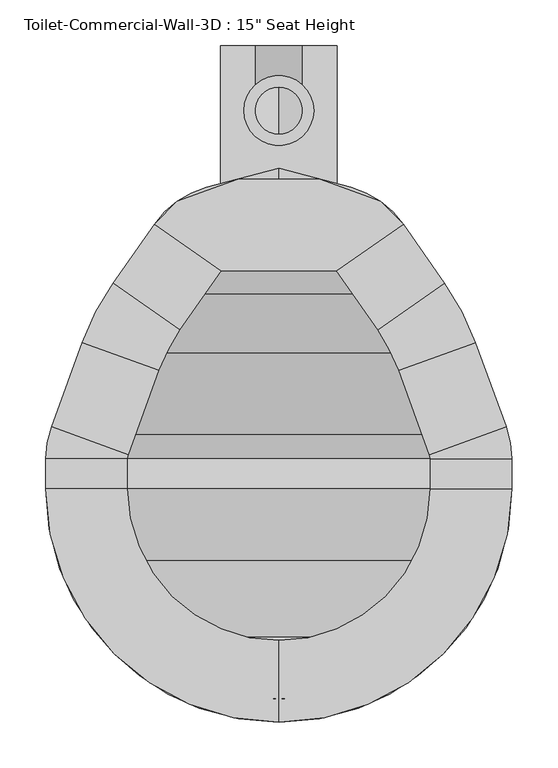
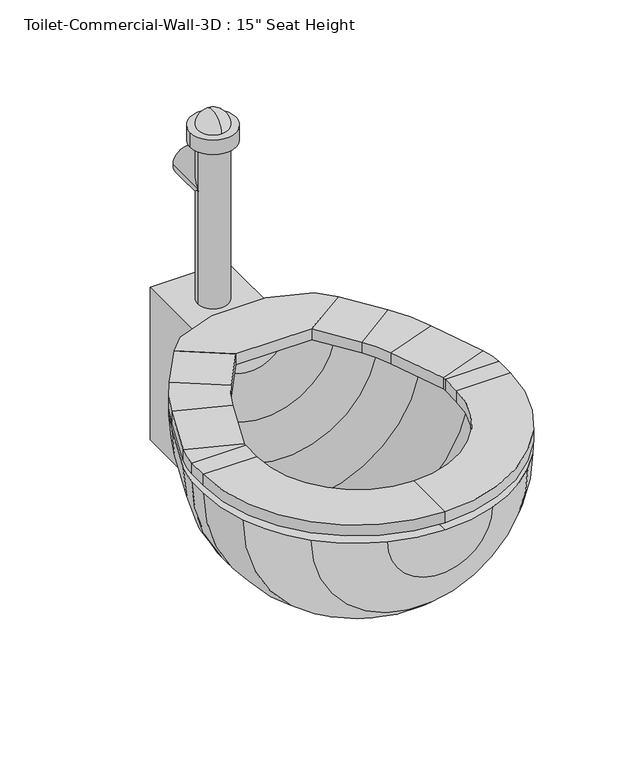
"""IFC4 building model written with IfcOpenShell, lengths in millimetres: flow terminal geometry."""

import ifcopenshell
import ifcopenshell.guid

model = None  # the IFC model being written
_history = None  # IfcOwnerHistory: only IFC2X3 demands one
_inside = {}  # id of a spatial element -> (the spatial element, [elements in it])
_under = {}  # id of a project, library or spatial element -> (it, [spatial elements below it])
_declared = {}  # id of a project -> (the project, [libraries it declares])
_typed = {}  # id of a type object -> (the type object, [elements of that type])
_made_of = {}  # id of a material, layer set ... -> (it, [elements and type objects made of it])


def new_model(schema):
    """Start an empty IFC model of exactly this schema.

    Asked for "IFC4X3", IfcOpenShell would pick the latest addendum, in which some entities
    have other attributes; the version numbers below select the first issue.
    IFC2X3 requires an IfcOwnerHistory on every rooted entity: one is made here for all.
    """
    global model, _history
    if schema == "IFC4X3":
        model = ifcopenshell.file(schema_version=(4, 3, 0, 0))
    else:
        model = ifcopenshell.file(schema=schema)
    _inside.clear()
    _under.clear()
    _declared.clear()
    _typed.clear()
    _made_of.clear()
    _history = None
    if model.schema == "IFC2X3":
        org = make("IfcOrganization", Name="unknown")
        user = make(
            "IfcPersonAndOrganization",
            ThePerson=make("IfcPerson", FamilyName="unknown"),
            TheOrganization=org,
        )
        app = make(
            "IfcApplication",
            ApplicationDeveloper=org,
            Version="unknown",
            ApplicationFullName="unknown",
            ApplicationIdentifier="unknown",
        )
        _history = make(
            "IfcOwnerHistory",
            OwningUser=user,
            OwningApplication=app,
            ChangeAction="ADDED",
            CreationDate=0,
        )
    return model


def make(cls, **values):
    """One entity of the class cls with the attributes given. An attribute that is None is left unset."""
    return model.create_entity(
        cls, **{name: value for name, value in values.items() if value is not None}
    )


def rooted(cls, **values):
    """An entity with a GlobalId (a new one), such as an element, a storey or a relation."""
    return make(cls, GlobalId=ifcopenshell.guid.new(), OwnerHistory=_history, **values)


def si_unit(unit_type, name, prefix=None):
    """IfcSIUnit, for example si_unit("LENGTHUNIT", "METRE", prefix="MILLI")."""
    return make("IfcSIUnit", UnitType=unit_type, Prefix=prefix, Name=name)


def assignment(units):
    """IfcUnitAssignment: the units of a project."""
    return None if units is None else make("IfcUnitAssignment", Units=units)


def point(xyz):
    """IfcCartesianPoint."""
    return None if xyz is None else make("IfcCartesianPoint", Coordinates=xyz)


def direction(xyz):
    """IfcDirection."""
    return None if xyz is None else make("IfcDirection", DirectionRatios=xyz)


def frame(location, z_axis=None, x_axis=None):
    """IfcAxis2Placement3D, a coordinate frame: its origin and axes. An axis left out is left unset."""
    return make(
        "IfcAxis2Placement3D",
        Location=point(location),
        Axis=direction(z_axis),
        RefDirection=direction(x_axis),
    )


def frame_2d(location, x_axis=None):
    """IfcAxis2Placement2D, a coordinate frame in the plane: its origin and x axis."""
    return make(
        "IfcAxis2Placement2D", Location=point(location), RefDirection=direction(x_axis)
    )


def origin():
    """The frame at (0, 0, 0) with its axes left unset."""
    return frame((0.0, 0.0, 0.0))


def place(relative_to, where):
    """IfcLocalPlacement: puts the frame where relative to a parent placement (None: the world)."""
    return make(
        "IfcLocalPlacement", PlacementRelTo=relative_to, RelativePlacement=where
    )


def context(
    kind, dimensions, precision=None, world=None, true_north=None, identifier=None
):
    """IfcGeometricRepresentationContext, for example the 3D "Model" context."""
    return make(
        "IfcGeometricRepresentationContext",
        ContextIdentifier=identifier,
        ContextType=kind,
        CoordinateSpaceDimension=dimensions,
        Precision=precision,
        WorldCoordinateSystem=world,
        TrueNorth=true_north,
    )


def project(units=None, contexts=None):
    """IfcProject with its units and contexts."""
    return rooted(
        "IfcProject",
        Name="project",
        RepresentationContexts=contexts,
        UnitsInContext=assignment(units),
    )


def spatial(cls, under=None, at=None, **own):
    """A site, building, storey or space (cls), placed at a placement, below another one or the project."""
    s = rooted(cls, ObjectPlacement=at, **own)
    if under is not None:
        _under.setdefault(under.id(), (under, []))[1].append(s)
    return s


def polyline(points):
    """IfcPolyline through the points."""
    return make("IfcPolyline", Points=[point(p) for p in points])


def circle_curve(where, radius):
    """IfcCircle in the frame where."""
    return make("IfcCircle", Position=where, Radius=radius)


def ellipse_curve(where, semi_axis1, semi_axis2):
    """IfcEllipse in the frame where."""
    return make(
        "IfcEllipse", Position=where, SemiAxis1=semi_axis1, SemiAxis2=semi_axis2
    )


def trimmed(basis, trim1, trim2, sense, master):
    """IfcTrimmedCurve: the piece of a basis curve between two trims."""
    return make(
        "IfcTrimmedCurve",
        BasisCurve=basis,
        Trim1=trim1,
        Trim2=trim2,
        SenseAgreement=sense,
        MasterRepresentation=master,
    )


def segment(curve, same_sense, transition):
    """IfcCompositeCurveSegment."""
    return make(
        "IfcCompositeCurveSegment",
        Transition=transition,
        SameSense=same_sense,
        ParentCurve=curve,
    )


def composite_curve(segments, self_intersect=None):
    """IfcCompositeCurve: segments joined end to end."""
    return make("IfcCompositeCurve", Segments=segments, SelfIntersect=self_intersect)


def outline(outer, holes=None, kind="AREA"):
    """IfcArbitraryClosedProfileDef: a profile drawn as a closed curve; with holes, ...WithVoids."""
    if holes is None:
        return make("IfcArbitraryClosedProfileDef", ProfileType=kind, OuterCurve=outer)
    return make(
        "IfcArbitraryProfileDefWithVoids",
        ProfileType=kind,
        OuterCurve=outer,
        InnerCurves=holes,
    )


def extrude(swept, where, along, depth):
    """IfcExtrudedAreaSolid: the profile swept, set in the frame where, extruded along a direction by depth."""
    return make(
        "IfcExtrudedAreaSolid",
        SweptArea=swept,
        Position=where,
        ExtrudedDirection=direction(along),
        Depth=depth,
    )


def shape(context_of_items, identifier, shape_type, items):
    """IfcShapeRepresentation: the items that make up one representation, for example the "Body"."""
    return make(
        "IfcShapeRepresentation",
        ContextOfItems=context_of_items,
        RepresentationIdentifier=identifier,
        RepresentationType=shape_type,
        Items=items,
    )


def source(mapping_origin, context_of_items, identifier, shape_type, items):
    """IfcRepresentationMap: a shape defined once, which mapped items show again and again."""
    return make(
        "IfcRepresentationMap",
        MappingOrigin=mapping_origin,
        MappedRepresentation=shape(context_of_items, identifier, shape_type, items),
    )


def transform(
    local_origin,
    x_axis=None,
    y_axis=None,
    z_axis=None,
    scale=None,
    scale2=None,
    scale3=None,
    uniform=True,
):
    """IfcCartesianTransformationOperator3D, or its non-uniform kind. x_axis, y_axis, z_axis: its Axis1, 2, 3."""
    if uniform:
        return make(
            "IfcCartesianTransformationOperator3D",
            Axis1=direction(x_axis),
            Axis2=direction(y_axis),
            LocalOrigin=point(local_origin),
            Scale=scale,
            Axis3=direction(z_axis),
        )
    return make(
        "IfcCartesianTransformationOperator3DnonUniform",
        Axis1=direction(x_axis),
        Axis2=direction(y_axis),
        LocalOrigin=point(local_origin),
        Scale=scale,
        Axis3=direction(z_axis),
        Scale2=scale2,
        Scale3=scale3,
    )


def mapped(mapping_source, mapping_target):
    """IfcMappedItem: shows the shape of a source again, moved by a transform."""
    return make(
        "IfcMappedItem", MappingSource=mapping_source, MappingTarget=mapping_target
    )


def made_of(thing, what):
    """Note that an element or type object is made of a material, layer set ...; save() writes the relation."""
    if what is not None:
        _made_of.setdefault(what.id(), (what, []))[1].append(thing)
    return thing


def element(
    cls,
    number,
    at=None,
    inside=None,
    cuts=None,
    type_object=None,
    material=None,
    context=None,
    identifier="Body",
    shape_type=None,
    held_by="IfcProductDefinitionShape",
    body=None,
    shapes=None,
    **own,
):
    """One element of the class cls, such as IfcWall. Its Tag is "e" and its number.

    at: its placement. inside: the storey or other place that contains it. cuts: it is an
    opening in that element (IfcRelVoidsElement). A single representation is given by context,
    identifier, shape_type and body (its items); several are given by shapes. held_by: the class
    of the entity that holds the representations. save() writes the other relations.
    """
    e = rooted(cls, Tag="e%d" % number, ObjectPlacement=at, **own)
    if body is not None:
        shapes = [shape(context, identifier, shape_type, body)]
    if shapes is not None:
        e.Representation = make(held_by, Representations=shapes)
    if inside is not None:
        _inside.setdefault(inside.id(), (inside, []))[1].append(e)
    if cuts is not None:
        rooted(
            "IfcRelVoidsElement", RelatingBuildingElement=cuts, RelatedOpeningElement=e
        )
    if type_object is not None:
        _typed.setdefault(type_object.id(), (type_object, []))[1].append(e)
    return made_of(e, material)


def aggregate(whole, parts):
    """IfcRelAggregates: a whole, such as a stair, and the parts it consists of."""
    return rooted("IfcRelAggregates", RelatingObject=whole, RelatedObjects=parts)


def save(model, path):
    """Write the relations noted so far, then the file.

    IfcRelAggregates (storeys below a building ...), IfcRelContainedInSpatialStructure (elements
    in a storey), IfcRelDefinesByType, IfcRelAssociatesMaterial and IfcRelDeclares: one each for
    every whole, place, type object, material and project.
    """
    for whole, parts in _under.values():
        aggregate(whole, parts)
    for where, things in _inside.values():
        rooted(
            "IfcRelContainedInSpatialStructure",
            RelatedElements=things,
            RelatingStructure=where,
        )
    for kind, things in _typed.values():
        rooted("IfcRelDefinesByType", RelatedObjects=things, RelatingType=kind)
    for what, things in _made_of.values():
        rooted("IfcRelAssociatesMaterial", RelatedObjects=things, RelatingMaterial=what)
    for by, libraries in _declared.values():
        rooted("IfcRelDeclares", RelatingContext=by, RelatedDefinitions=libraries)
    model.write(path)


def plane_surface(at):
    """IfcPlane: the flat surface through the origin of the frame at, square to its z axis."""
    return make("IfcPlane", Position=at)


def cylinder_surface(at, radius):
    """IfcCylindricalSurface: all points at the distance radius from the z axis of the frame at."""
    return make("IfcCylindricalSurface", Position=at, Radius=radius)


def revolved_surface(curve, axis_point, axis_direction):
    """IfcSurfaceOfRevolution: the curve turned about the line through axis_point along axis_direction."""
    return make(
        "IfcSurfaceOfRevolution",
        SweptCurve=make("IfcArbitraryOpenProfileDef", ProfileType="CURVE", Curve=curve),
        AxisPosition=make("IfcAxis1Placement", Location=point(axis_point), Axis=direction(axis_direction)),
    )


def advanced_brep(points, edges, surfaces, faces):
    """IfcAdvancedBrep: a solid bounded by faces that lie on surfaces and meet in shared edges.

    An edge is (start, end): straight between two places in points (the first is 0);
    or (start, end, curve); or (start, end, curve, False) where it runs against its curve.
    A face is (place in surfaces, loops), or (place, loops, False) where it looks against
    its surface's normal. A loop lists edges by number (the first is 1), with a minus sign
    where the edge is run from its end to its start. The first loop is the outer one.
    """
    corners = [point(p) for p in points]
    vertices = [make("IfcVertexPoint", VertexGeometry=c) for c in corners]
    made = []
    for start, end, *more in edges:
        made.append(
            make(
                "IfcEdgeCurve",
                EdgeStart=vertices[start],
                EdgeEnd=vertices[end],
                EdgeGeometry=more[0] if more else make("IfcPolyline", Points=[corners[start], corners[end]]),
                SameSense=more[1] if len(more) > 1 else True,
            )
        )
    hull = []
    for where, loops, *sense in faces:
        bounds = []
        for j, loop in enumerate(loops):
            ring = [make("IfcOrientedEdge", EdgeElement=made[abs(k) - 1], Orientation=k > 0) for k in loop]
            bounds.append(
                make(
                    "IfcFaceOuterBound" if j == 0 else "IfcFaceBound",
                    Bound=make("IfcEdgeLoop", EdgeList=ring),
                    Orientation=True,
                )
            )
        hull.append(make("IfcAdvancedFace", Bounds=bounds, FaceSurface=surfaces[where], SameSense=sense[0] if sense else True))
    return make("IfcAdvancedBrep", Outer=make("IfcClosedShell", CfsFaces=hull))


def flow_terminal_62e3d79f(model_context):
    return source(origin(), model_context, "Body", "SolidModel", [
        extrude(outline(polyline([(467.7541169, -443.4722495), (342.0521907, -443.4722495), (269.229574, -392.4813043), (294.1800557, -367.5308226), (360.2423986, -343.4860961), (449.563909, -343.4860961), (515.6262519, -367.5308226), (540.5767337, -392.4813043), (467.7541169, -443.4722495)])), frame((0.0, 0.0, 355.6), z_axis=(0.0, 0.0, 1.0), x_axis=(1.0, 0.0, 0.0)), (0.0, 0.0, 1.0), 19.05),
        advanced_brep(
        [(467.7541169, -443.4722495, 355.6), (467.7541169, -443.4722495, 374.65), (540.5767337, -392.4813043, 374.65), (540.5767337, -392.4813043, 355.6), (585.6810159, -456.8968951, 355.6), (512.8583992, -507.8878403, 355.6), (585.6810159, -456.8968951, 374.65), (512.8583992, -507.8878403, 374.65), (619.360053, -521.5937234, 355.6), (535.821379, -551.9993141, 355.6), (619.360053, -521.5937234, 374.65), (535.821379, -551.9993141, 374.65), (652.7759241, -613.4030747, 355.6), (569.2372501, -643.8086654, 355.6), (652.7759241, -613.4030747, 374.65), (569.2372501, -643.8086654, 374.65), (658.9031538, -648.1523212, 355.6), (570.0031538, -648.1523212, 355.6), (658.9031538, -648.1523212, 374.65), (570.0031538, -648.1523212, 374.65), (658.9031538, -681.0375, 355.6), (570.0031538, -681.0375, 355.6), (658.9031538, -681.0375, 374.65), (570.0031538, -681.0375, 374.65), (404.9031538, -935.0375, 355.6), (404.9031538, -846.1375, 355.6), (404.9031538, -935.0375, 374.65), (404.9031538, -846.1375, 374.65), (150.9031538, -681.0375, 355.6), (239.8031538, -681.0375, 355.6), (150.9031538, -681.0375, 374.65), (239.8031538, -681.0375, 374.65), (150.9031538, -648.1523212, 355.6), (239.8031538, -648.1523212, 355.6), (150.9031538, -648.1523212, 374.65), (239.8031538, -648.1523212, 374.65), (157.0303835, -613.4030747, 355.6), (240.5690575, -643.8086654, 355.6), (157.0303835, -613.4030747, 374.65), (240.5690575, -643.8086654, 374.65), (190.4462546, -521.5937234, 355.6), (273.9849286, -551.9993141, 355.6), (190.4462546, -521.5937234, 374.65), (273.9849286, -551.9993141, 374.65), (224.1252917, -456.8968951, 355.6), (296.9479084, -507.8878403, 355.6), (224.1252917, -456.8968951, 374.65), (296.9479084, -507.8878403, 374.65), (342.0521907, -443.4722495, 355.6), (269.229574, -392.4813043, 355.6), (269.229574, -392.4813043, 374.65), (342.0521907, -443.4722495, 374.65)],
        [
            (0, 1),
            (1, 2),
            (2, 3),
            (3, 0),
            (3, 4),
            (4, 5),
            (5, 0),
            (2, 6),
            (6, 4),
            (1, 7),
            (7, 6),
            (5, 7),
            (8, 9),
            (9, 5, circle_curve(frame((356.8099347, -617.1541514, 355.6), z_axis=(0.0, 0.0, 1.0), x_axis=(0.81915204428899, 0.5735764363510486, 0.0)), 190.5)),
            (4, 8, circle_curve(frame((356.8099347, -617.1541514, 355.6), z_axis=(0.0, 0.0, -1.0), x_axis=(0.81915204428899, 0.5735764363510486, 0.0)), 279.4)),
            (10, 8),
            (6, 10, circle_curve(frame((356.8099347, -617.1541514, 374.65), z_axis=(0.0, 0.0, -1.0), x_axis=(0.81915204428899, 0.5735764363510486, 0.0)), 279.4)),
            (11, 10),
            (7, 11, circle_curve(frame((356.8099347, -617.1541514, 374.65), z_axis=(0.0, 0.0, -1.0), x_axis=(0.81915204428899, 0.5735764363510486, 0.0)), 190.5)),
            (9, 11),
            (8, 12),
            (12, 13),
            (13, 9),
            (10, 14),
            (14, 12),
            (11, 15),
            (15, 14),
            (13, 15),
            (16, 17),
            (17, 13, circle_curve(frame((557.3031538, -648.1523212, 355.6), z_axis=(0.0, 0.0, 1.0), x_axis=(0.9396926207859057, 0.3420201433256761, 0.0)), 12.7)),
            (12, 16, circle_curve(frame((557.3031538, -648.1523212, 355.6), z_axis=(0.0, 0.0, -1.0), x_axis=(0.9396926207859057, 0.3420201433256761, 0.0)), 101.6)),
            (18, 16),
            (14, 18, circle_curve(frame((557.3031538, -648.1523212, 374.65), z_axis=(0.0, 0.0, -1.0), x_axis=(0.9396926207859057, 0.3420201433256761, 0.0)), 101.6)),
            (19, 18),
            (15, 19, circle_curve(frame((557.3031538, -648.1523212, 374.65), z_axis=(0.0, 0.0, -1.0), x_axis=(0.9396926207859057, 0.3420201433256761, 0.0)), 12.7)),
            (17, 19),
            (16, 20),
            (20, 21),
            (21, 17),
            (18, 22),
            (22, 20),
            (19, 23),
            (23, 22),
            (21, 23),
            (24, 25),
            (25, 21, circle_curve(frame((404.9031538, -681.0375, 355.6), z_axis=(0.0, 0.0, 1.0), x_axis=(1.0, 0.0, 0.0)), 165.1)),
            (20, 24, circle_curve(frame((404.9031538, -681.0375, 355.6), z_axis=(0.0, 0.0, -1.0), x_axis=(1.0, 0.0, 0.0)), 254.0)),
            (26, 24),
            (22, 26, circle_curve(frame((404.9031538, -681.0375, 374.65), z_axis=(0.0, 0.0, -1.0), x_axis=(1.0, 0.0, 0.0)), 254.0)),
            (27, 26),
            (23, 27, circle_curve(frame((404.9031538, -681.0375, 374.65), z_axis=(0.0, 0.0, -1.0), x_axis=(1.0, 0.0, 0.0)), 165.1)),
            (25, 27),
            (28, 29),
            (29, 25, circle_curve(frame((404.9031538, -681.0375, 355.6), z_axis=(0.0, 0.0, 1.0), x_axis=(0.0, -1.0, 0.0)), 165.1)),
            (24, 28, circle_curve(frame((404.9031538, -681.0375, 355.6), z_axis=(0.0, 0.0, -1.0), x_axis=(0.0, -1.0, 0.0)), 254.0)),
            (30, 28),
            (26, 30, circle_curve(frame((404.9031538, -681.0375, 374.65), z_axis=(0.0, 0.0, -1.0), x_axis=(0.0, -1.0, 0.0)), 254.0)),
            (31, 30),
            (27, 31, circle_curve(frame((404.9031538, -681.0375, 374.65), z_axis=(0.0, 0.0, -1.0), x_axis=(0.0, -1.0, 0.0)), 165.1)),
            (29, 31),
            (28, 32),
            (32, 33),
            (33, 29),
            (30, 34),
            (34, 32),
            (31, 35),
            (35, 34),
            (33, 35),
            (36, 37),
            (37, 33, circle_curve(frame((252.5031538, -648.1523212, 355.6), z_axis=(0.0, 0.0, 1.0), x_axis=(-1.0, 0.0, 0.0)), 12.7)),
            (32, 36, circle_curve(frame((252.5031538, -648.1523212, 355.6), z_axis=(0.0, 0.0, -1.0), x_axis=(-1.0, 0.0, 0.0)), 101.6)),
            (38, 36),
            (34, 38, circle_curve(frame((252.5031538, -648.1523212, 374.65), z_axis=(0.0, 0.0, -1.0), x_axis=(-1.0, 0.0, 0.0)), 101.6)),
            (39, 38),
            (35, 39, circle_curve(frame((252.5031538, -648.1523212, 374.65), z_axis=(0.0, 0.0, -1.0), x_axis=(-1.0, 0.0, 0.0)), 12.7)),
            (37, 39),
            (36, 40),
            (40, 41),
            (41, 37),
            (38, 42),
            (42, 40),
            (39, 43),
            (43, 42),
            (41, 43),
            (44, 45),
            (45, 41, circle_curve(frame((452.9963729, -617.1541514, 355.6), z_axis=(0.0, 0.0, 1.0), x_axis=(-0.939692620785909, 0.3420201433256672, 0.0)), 190.5)),
            (40, 44, circle_curve(frame((452.9963729, -617.1541514, 355.6), z_axis=(0.0, 0.0, -1.0), x_axis=(-0.939692620785909, 0.3420201433256672, 0.0)), 279.4)),
            (46, 44),
            (42, 46, circle_curve(frame((452.9963729, -617.1541514, 374.65), z_axis=(0.0, 0.0, -1.0), x_axis=(-0.939692620785909, 0.3420201433256672, 0.0)), 279.4)),
            (47, 46),
            (43, 47, circle_curve(frame((452.9963729, -617.1541514, 374.65), z_axis=(0.0, 0.0, -1.0), x_axis=(-0.939692620785909, 0.3420201433256672, 0.0)), 190.5)),
            (45, 47),
            (48, 49),
            (49, 50),
            (50, 51),
            (51, 48),
            (44, 49),
            (48, 45),
            (46, 50),
            (47, 51),
        ],
        [
            plane_surface(frame((540.5767337, -392.4813043, 437.2995365), z_axis=(-0.5735764363510436, 0.8191520442889937, 0.0), x_axis=(0.8191520442889937, 0.5735764363510436, 0.0))),
            plane_surface(frame((467.7541169, -443.4722495, 355.6), z_axis=(0.0, 0.0, -1.0), x_axis=(0.5735764363510436, -0.8191520442889936, 0.0))),
            plane_surface(frame((540.5767337, -392.4813043, 355.6), z_axis=(0.8191520442889944, 0.5735764363510424, 0.0), x_axis=(0.5735764363510424, -0.8191520442889944, 0.0))),
            plane_surface(frame((540.5767337, -392.4813043, 374.65), z_axis=(0.0, 0.0, 1.0), x_axis=(0.573576436351043, -0.819152044288994, 0.0))),
            plane_surface(frame((467.7541169, -443.4722495, 374.65), z_axis=(-0.819152044288994, -0.573576436351043, 0.0), x_axis=(0.573576436351043, -0.819152044288994, 0.0))),
            plane_surface(frame((356.8099347, -617.1541514, 355.6), z_axis=(0.0, 0.0, -1.0), x_axis=(0.81915204428899, 0.5735764363510486, 0.0))),
            cylinder_surface(frame((356.8099347, -617.1541514, 342.9), z_axis=(0.0, 0.0, 1.0), x_axis=(0.81915204428899, 0.5735764363510486, 0.0)), 279.4),
            plane_surface(frame((356.8099347, -617.1541514, 374.65), z_axis=(0.0, 0.0, 1.0), x_axis=(0.81915204428899, 0.5735764363510486, 0.0))),
            revolved_surface(polyline([(512.8583991370526, -507.8878402751253, 374.65), (512.8583991370526, -507.8878402751253, 355.6)]), (356.8099347, -617.1541514, 342.9), (0.0, 0.0, 1.0)),
            plane_surface(frame((535.821379, -551.9993141, 355.6), z_axis=(0.0, 0.0, -1.0000000000000002), x_axis=(0.3420201433256594, -0.9396926207859119, 0.0))),
            plane_surface(frame((619.360053, -521.5937234, 355.6), z_axis=(0.9396926207859121, 0.3420201433256587, 0.0), x_axis=(0.3420201433256587, -0.9396926207859121, 0.0))),
            plane_surface(frame((619.360053, -521.5937234, 374.65), z_axis=(0.0, 0.0, 1.0), x_axis=(0.34202014332565916, -0.9396926207859119, 0.0))),
            plane_surface(frame((535.821379, -551.9993141, 374.65), z_axis=(-0.9396926207859122, -0.34202014332565833, 0.0), x_axis=(0.34202014332565833, -0.9396926207859122, 0.0))),
            plane_surface(frame((557.3031538, -648.1523212, 355.6), z_axis=(0.0, 0.0, -1.0000000000000002), x_axis=(0.9396926207859058, 0.34202014332567615, 0.0))),
            cylinder_surface(frame((557.3031538, -648.1523212, 342.9), z_axis=(0.0, 0.0, 1.0), x_axis=(0.9396926207859057, 0.3420201433256761, 0.0)), 101.6),
            plane_surface(frame((557.3031538, -648.1523212, 374.65), z_axis=(0.0, 0.0, 1.0000000000000002), x_axis=(0.9396926207859058, 0.34202014332567615, 0.0))),
            revolved_surface(polyline([(569.237250083981, -643.8086653797639, 374.65), (569.237250083981, -643.8086653797639, 355.6)]), (557.3031538, -648.1523212, 342.9), (0.0, 0.0, 1.0)),
            plane_surface(frame((570.0031538, -648.1523212, 355.6), z_axis=(0.0, 0.0, -1.0), x_axis=(0.0, -1.0, 0.0))),
            plane_surface(frame((658.9031538, -648.1523212, 355.6), z_axis=(1.0, 0.0, 0.0), x_axis=(0.0, -1.0, 0.0))),
            plane_surface(frame((658.9031538, -648.1523212, 374.65), z_axis=(0.0, 0.0, 1.0), x_axis=(0.0, -1.0, 0.0))),
            plane_surface(frame((570.0031538, -648.1523212, 374.65), z_axis=(-1.0, 0.0, 0.0), x_axis=(0.0, -1.0, 0.0))),
            plane_surface(frame((404.9031538, -681.0375, 355.6), z_axis=(0.0, 0.0, -1.0), x_axis=(1.0, 0.0, 0.0))),
            cylinder_surface(frame((404.9031538, -681.0375, 342.9), z_axis=(0.0, 0.0, 1.0), x_axis=(1.0, 0.0, 0.0)), 254.0),
            plane_surface(frame((404.9031538, -681.0375, 374.65), z_axis=(0.0, 0.0, 1.0), x_axis=(1.0, 0.0, 0.0))),
            revolved_surface(polyline([(570.0031538, -681.0375, 374.65), (570.0031538, -681.0375, 355.6)]), (404.9031538, -681.0375, 342.9), (0.0, 0.0, 1.0)),
            plane_surface(frame((404.9031538, -681.0375, 355.6), z_axis=(0.0, 0.0, -1.0), x_axis=(0.0, -1.0, 0.0))),
            cylinder_surface(frame((404.9031538, -681.0375, 342.9), z_axis=(0.0, 0.0, 1.0), x_axis=(0.0, -1.0, 0.0)), 254.0),
            plane_surface(frame((404.9031538, -681.0375, 374.65), z_axis=(0.0, 0.0, 1.0), x_axis=(0.0, -1.0, 0.0))),
            revolved_surface(polyline([(404.9031538, -846.1375, 374.65), (404.9031538, -846.1375, 355.6)]), (404.9031538, -681.0375, 342.9), (0.0, 0.0, 1.0)),
            plane_surface(frame((239.8031538, -681.0375, 355.6), z_axis=(0.0, 0.0, -1.0), x_axis=(0.0, 1.0, 0.0))),
            plane_surface(frame((150.9031538, -681.0375, 355.6), z_axis=(-1.0, 0.0, 0.0), x_axis=(0.0, 1.0, 0.0))),
            plane_surface(frame((150.9031538, -681.0375, 374.65), z_axis=(0.0, 0.0, 1.0), x_axis=(0.0, 1.0, 0.0))),
            plane_surface(frame((239.8031538, -681.0375, 374.65), z_axis=(1.0, 0.0, 0.0), x_axis=(0.0, 1.0, 0.0))),
            plane_surface(frame((252.5031538, -648.1523212, 355.6), z_axis=(0.0, 0.0, -1.0), x_axis=(-1.0, 0.0, 0.0))),
            cylinder_surface(frame((252.5031538, -648.1523212, 342.9), z_axis=(0.0, 0.0, 1.0), x_axis=(-1.0, 0.0, 0.0)), 101.6),
            plane_surface(frame((252.5031538, -648.1523212, 374.65), z_axis=(0.0, 0.0, 1.0), x_axis=(-1.0, 0.0, 0.0))),
            revolved_surface(polyline([(239.80315380000002, -648.1523212, 374.65), (239.80315380000002, -648.1523212, 355.6)]), (252.5031538, -648.1523212, 342.9), (0.0, 0.0, 1.0)),
            plane_surface(frame((240.5690575, -643.8086654, 355.6), z_axis=(0.0, 0.0, -1.0), x_axis=(0.3420201433256581, 0.9396926207859123, 0.0))),
            plane_surface(frame((157.0303835, -613.4030747, 355.6), z_axis=(-0.9396926207859122, 0.3420201433256583, 0.0), x_axis=(0.3420201433256583, 0.9396926207859122, 0.0))),
            plane_surface(frame((157.0303835, -613.4030747, 374.65), z_axis=(0.0, 0.0, 1.0), x_axis=(0.34202014332565855, 0.9396926207859121, 0.0))),
            plane_surface(frame((240.5690575, -643.8086654, 374.65), z_axis=(0.9396926207859124, -0.3420201433256579, 0.0), x_axis=(0.3420201433256579, 0.9396926207859124, 0.0))),
            plane_surface(frame((452.9963729, -617.1541514, 355.6), z_axis=(0.0, 0.0, -1.0), x_axis=(-0.939692620785909, 0.3420201433256672, 0.0))),
            cylinder_surface(frame((452.9963729, -617.1541514, 342.9), z_axis=(0.0, 0.0, 1.0), x_axis=(-0.939692620785909, 0.3420201433256672, 0.0)), 279.4),
            plane_surface(frame((452.9963729, -617.1541514, 374.65), z_axis=(0.0, 0.0, 1.0), x_axis=(-0.939692620785909, 0.3420201433256672, 0.0))),
            revolved_surface(polyline([(273.98492864028435, -551.9993140964605, 374.65), (273.98492864028435, -551.9993140964605, 355.6)]), (452.9963729, -617.1541514, 342.9), (0.0, 0.0, 1.0)),
            plane_surface(frame((269.229574, -392.4813043, 248.5004635), z_axis=(0.5735764363510469, 0.8191520442889914, 0.0), x_axis=(0.8191520442889914, -0.5735764363510469, 0.0))),
            plane_surface(frame((296.9479084, -507.8878403, 355.6), z_axis=(0.0, 0.0, -1.0), x_axis=(0.5735764363510465, 0.8191520442889916, 0.0))),
            plane_surface(frame((224.1252917, -456.8968951, 355.6), z_axis=(-0.819152044288991, 0.5735764363510473, 0.0), x_axis=(0.5735764363510473, 0.819152044288991, 0.0))),
            plane_surface(frame((224.1252917, -456.8968951, 374.65), z_axis=(0.0, 0.0, 1.0), x_axis=(0.5735764363510473, 0.819152044288991, 0.0))),
            plane_surface(frame((296.9479084, -507.8878403, 374.65), z_axis=(0.8191520442889914, -0.5735764363510468, 0.0), x_axis=(0.5735764363510468, 0.8191520442889914, 0.0))),
        ],
        [
            (0, [[1, 2, 3, 4]]),
            (1, [[5, 6, 7, -4]]),
            (2, [[8, 9, -5, -3]]),
            (3, [[10, 11, -8, -2]]),
            (4, [[-7, 12, -10, -1]]),
            (5, [[13, 14, -6, 15]]),
            (6, [[16, -15, -9, 17]]),
            (7, [[18, -17, -11, 19]]),
            (8, [[20, -19, -12, -14]]),
            (9, [[21, 22, 23, -13]]),
            (10, [[24, 25, -21, -16]]),
            (11, [[26, 27, -24, -18]]),
            (12, [[-23, 28, -26, -20]]),
            (13, [[29, 30, -22, 31]]),
            (14, [[32, -31, -25, 33]]),
            (15, [[34, -33, -27, 35]]),
            (16, [[36, -35, -28, -30]]),
            (17, [[37, 38, 39, -29]]),
            (18, [[40, 41, -37, -32]]),
            (19, [[42, 43, -40, -34]]),
            (20, [[-39, 44, -42, -36]]),
            (21, [[45, 46, -38, 47]]),
            (22, [[48, -47, -41, 49]]),
            (23, [[50, -49, -43, 51]]),
            (24, [[52, -51, -44, -46]]),
            (25, [[53, 54, -45, 55]]),
            (26, [[56, -55, -48, 57]]),
            (27, [[58, -57, -50, 59]]),
            (28, [[60, -59, -52, -54]]),
            (29, [[61, 62, 63, -53]]),
            (30, [[64, 65, -61, -56]]),
            (31, [[66, 67, -64, -58]]),
            (32, [[-63, 68, -66, -60]]),
            (33, [[69, 70, -62, 71]]),
            (34, [[72, -71, -65, 73]]),
            (35, [[74, -73, -67, 75]]),
            (36, [[76, -75, -68, -70]]),
            (37, [[77, 78, 79, -69]]),
            (38, [[80, 81, -77, -72]]),
            (39, [[82, 83, -80, -74]]),
            (40, [[-79, 84, -82, -76]]),
            (41, [[85, 86, -78, 87]]),
            (42, [[88, -87, -81, 89]]),
            (43, [[90, -89, -83, 91]]),
            (44, [[92, -91, -84, -86]]),
            (45, [[93, 94, 95, 96]]),
            (46, [[97, -93, 98, -85]]),
            (47, [[99, -94, -97, -88]]),
            (48, [[100, -95, -99, -90]]),
            (49, [[-98, -96, -100, -92]]),
        ],
    ),
        advanced_brep(
        [(491.7762702, -919.7194257, 342.9), (584.5082762, -860.6426224, 342.9), (643.5850795, -767.9106164, 342.9), (658.9031538, -681.0375, 342.9), (658.9031538, -648.1523212, 342.9), (652.7759241, -613.4030747, 342.9), (619.360053, -521.5937234, 342.9), (585.6810159, -456.8968951, 342.9), (540.5767337, -392.4813043, 342.9), (483.6469009, -352.6186063, 342.9), (404.9031538, -331.5192829, 342.9), (404.9031538, -357.8152978, 342.9), (468.1430637, -374.7603806, 342.9), (525.0728964, -414.6230786, 342.9), (562.9565296, -468.7265139, 342.9), (596.6355667, -533.4233422, 342.9), (628.9077315, -622.0903863, 342.9), (633.5031538, -648.1523212, 342.9), (633.5031538, -681.0375, 342.9), (619.7168869, -759.2233048, 342.9), (566.547764, -842.6821102, 342.9), (483.0889586, -895.8512331, 342.9), (404.9031538, -909.6375, 342.9), (404.9031538, -935.0375, 342.9), (318.0300374, -919.7194257, 342.9), (326.7173491, -895.8512331, 342.9), (243.2585436, -842.6821102, 342.9), (190.0894207, -759.2233048, 342.9), (176.3031538, -681.0375, 342.9), (176.3031538, -648.1523212, 342.9), (180.8985761, -622.0903863, 342.9), (213.1707409, -533.4233422, 342.9), (246.849778, -468.7265139, 342.9), (284.7334112, -414.6230786, 342.9), (341.663244, -374.7603806, 342.9), (326.1594067, -352.6186063, 342.9), (269.229574, -392.4813043, 342.9), (224.1252917, -456.8968951, 342.9), (190.4462546, -521.5937234, 342.9), (157.0303835, -613.4030747, 342.9), (150.9031538, -648.1523212, 342.9), (150.9031538, -681.0375, 342.9), (166.2212281, -767.9106164, 342.9), (225.2980314, -860.6426224, 342.9)],
        [
            (0, 1, circle_curve(frame((404.9031538, -681.0375, 342.9), z_axis=(0.0, 0.0, 1.0), x_axis=(1.0, 0.0, 0.0)), 254.0)),
            (1, 2, circle_curve(frame((404.9031538, -681.0375, 342.9), z_axis=(0.0, 0.0, 1.0), x_axis=(1.0, 0.0, 0.0)), 254.0)),
            (2, 3, circle_curve(frame((404.9031538, -681.0375, 342.9), z_axis=(0.0, 0.0, 1.0), x_axis=(1.0, 0.0, 0.0)), 254.0)),
            (3, 4),
            (4, 5, circle_curve(frame((557.3031538, -648.1523212, 342.9), z_axis=(0.0, 0.0, 1.0), x_axis=(1.0, 0.0, 0.0)), 101.6)),
            (5, 6),
            (6, 7, circle_curve(frame((356.8099347, -617.1541514, 342.9), z_axis=(0.0, 0.0, 1.0), x_axis=(1.0, 0.0, 0.0)), 279.4)),
            (7, 8),
            (8, 9, circle_curve(frame((457.350886, -450.7566703, 342.9), z_axis=(0.0, 0.0, 1.0), x_axis=(1.0, 0.0, 0.0)), 101.6)),
            (9, 10),
            (10, 11),
            (11, 12),
            (12, 13, circle_curve(frame((441.8470487, -472.8984446, 342.9), z_axis=(0.0, 0.0, -1.0), x_axis=(1.0, 0.0, 0.0)), 101.6)),
            (13, 14),
            (14, 15, circle_curve(frame((334.0854485, -628.9837703, 342.9), z_axis=(0.0, 0.0, -1.0), x_axis=(1.0, 0.0, 0.0)), 279.4)),
            (15, 16),
            (16, 17, circle_curve(frame((557.3031538, -648.1523212, 342.9), z_axis=(0.0, 0.0, -1.0), x_axis=(1.0, 0.0, 0.0)), 76.2)),
            (17, 18),
            (18, 19, circle_curve(frame((404.9031538, -681.0375, 342.9), z_axis=(0.0, 0.0, -1.0), x_axis=(1.0, 0.0, 0.0)), 228.6)),
            (19, 20, circle_curve(frame((404.9031538, -681.0375, 342.9), z_axis=(0.0, 0.0, -1.0), x_axis=(1.0, 0.0, 0.0)), 228.6)),
            (20, 21, circle_curve(frame((404.9031538, -681.0375, 342.9), z_axis=(0.0, 0.0, -1.0), x_axis=(1.0, 0.0, 0.0)), 228.6)),
            (21, 22, circle_curve(frame((404.9031538, -681.0375, 342.9), z_axis=(0.0, 0.0, -1.0), x_axis=(1.0, 0.0, 0.0)), 228.6)),
            (22, 23),
            (23, 0, circle_curve(frame((404.9031538, -681.0375, 342.9), z_axis=(0.0, 0.0, 1.0), x_axis=(1.0, 0.0, 0.0)), 254.0)),
            (24, 23, circle_curve(frame((404.9031538, -681.0375, 342.9), z_axis=(0.0, 0.0, 1.0), x_axis=(-1.0, 0.0, 0.0)), 254.0)),
            (22, 25, circle_curve(frame((404.9031538, -681.0375, 342.9), z_axis=(0.0, 0.0, -1.0), x_axis=(-1.0, 0.0, 0.0)), 228.6)),
            (25, 26, circle_curve(frame((404.9031538, -681.0375, 342.9), z_axis=(0.0, 0.0, -1.0), x_axis=(-1.0, 0.0, 0.0)), 228.6)),
            (26, 27, circle_curve(frame((404.9031538, -681.0375, 342.9), z_axis=(0.0, 0.0, -1.0), x_axis=(-1.0, 0.0, 0.0)), 228.6)),
            (27, 28, circle_curve(frame((404.9031538, -681.0375, 342.9), z_axis=(0.0, 0.0, -1.0), x_axis=(-1.0, 0.0, 0.0)), 228.6)),
            (28, 29),
            (29, 30, circle_curve(frame((252.5031538, -648.1523212, 342.9), z_axis=(0.0, 0.0, -1.0), x_axis=(-1.0, 0.0, 0.0)), 76.2)),
            (30, 31),
            (31, 32, circle_curve(frame((475.7208592, -628.9837703, 342.9), z_axis=(0.0, 0.0, -1.0), x_axis=(-1.0, 0.0, 0.0)), 279.4)),
            (32, 33),
            (33, 34, circle_curve(frame((367.9592589, -472.8984446, 342.9), z_axis=(0.0, 0.0, -1.0), x_axis=(-1.0, 0.0, 0.0)), 101.6)),
            (34, 11),
            (10, 35),
            (35, 36, circle_curve(frame((352.4554217, -450.7566703, 342.9), z_axis=(0.0, 0.0, 1.0), x_axis=(-1.0, 0.0, 0.0)), 101.6)),
            (36, 37),
            (37, 38, circle_curve(frame((452.9963729, -617.1541514, 342.9), z_axis=(0.0, 0.0, 1.0), x_axis=(-1.0, 0.0, 0.0)), 279.4)),
            (38, 39),
            (39, 40, circle_curve(frame((252.5031538, -648.1523212, 342.9), z_axis=(0.0, 0.0, 1.0), x_axis=(-1.0, 0.0, 0.0)), 101.6)),
            (40, 41),
            (41, 42, circle_curve(frame((404.9031538, -681.0375, 342.9), z_axis=(0.0, 0.0, 1.0), x_axis=(-1.0, 0.0, 0.0)), 254.0)),
            (42, 43, circle_curve(frame((404.9031538, -681.0375, 342.9), z_axis=(0.0, 0.0, 1.0), x_axis=(-1.0, 0.0, 0.0)), 254.0)),
            (43, 24, circle_curve(frame((404.9031538, -681.0375, 342.9), z_axis=(0.0, 0.0, 1.0), x_axis=(-1.0, 0.0, 0.0)), 254.0)),
            (24, 0, circle_curve(frame((404.9031538, -919.7194257, 342.9), z_axis=(0.0, -1.0, 0.0), x_axis=(1.0, 0.0, 0.0)), 86.8731164)),
            (21, 25, circle_curve(frame((404.9031538, -895.8512331, 342.9), z_axis=(0.0, 1.0, 0.0), x_axis=(1.0, 0.0, 0.0)), 78.1858048)),
            (20, 26, circle_curve(frame((404.9031538, -842.6821102, 342.9), z_axis=(0.0, 1.0, 0.0), x_axis=(1.0, 0.0, 0.0)), 161.6446102)),
            (19, 27, circle_curve(frame((404.9031538, -759.2233048, 342.9), z_axis=(0.0, 1.0, 0.0), x_axis=(1.0, 0.0, 0.0)), 214.8137331)),
            (18, 28, circle_curve(frame((404.9031538, -681.0375, 342.9), z_axis=(0.0, 1.0, 0.0), x_axis=(1.0, 0.0, 0.0)), 228.6)),
            (17, 29, circle_curve(frame((404.9031538, -648.1523212, 342.9), z_axis=(0.0, 1.0, 0.0), x_axis=(1.0, 0.0, 0.0)), 228.6)),
            (16, 30, circle_curve(frame((404.9031538, -622.0903863, 342.9), z_axis=(0.0, 1.0, 0.0), x_axis=(1.0, 0.0, 0.0)), 224.0045777)),
            (15, 31, circle_curve(frame((404.9031538, -533.4233422, 342.9), z_axis=(0.0, 1.0, 0.0), x_axis=(1.0, 0.0, 0.0)), 191.7324129)),
            (14, 32, circle_curve(frame((404.9031538, -468.7265139, 342.9), z_axis=(0.0, 1.0, 0.0), x_axis=(1.0, 0.0, 0.0)), 158.0533758)),
            (13, 33, circle_curve(frame((404.9031538, -414.6230786, 342.9), z_axis=(0.0, 1.0, 0.0), x_axis=(1.0, 0.0, 0.0)), 120.1697426)),
            (12, 34, circle_curve(frame((404.9031538, -374.7603806, 342.9), z_axis=(0.0, 1.0, 0.0), x_axis=(1.0, 0.0, 0.0)), 63.2399099)),
            (9, 35, circle_curve(frame((404.9031538, -352.6186063, 342.9), z_axis=(0.0, 1.0, 0.0), x_axis=(1.0, 0.0, 0.0)), 78.7437471)),
            (8, 36, circle_curve(frame((404.9031538, -392.4813043, 342.9), z_axis=(0.0, 1.0, 0.0), x_axis=(1.0, 0.0, 0.0)), 135.6735798)),
            (7, 37, circle_curve(frame((404.9031538, -456.8968951, 342.9), z_axis=(0.0, 1.0, 0.0), x_axis=(1.0, 0.0, 0.0)), 180.7778621)),
            (6, 38, circle_curve(frame((404.9031538, -521.5937234, 342.9), z_axis=(0.0, 1.0, 0.0), x_axis=(1.0, 0.0, 0.0)), 214.4568992)),
            (5, 39, circle_curve(frame((404.9031538, -613.4030747, 342.9), z_axis=(0.0, 1.0, 0.0), x_axis=(1.0, 0.0, 0.0)), 247.8727703)),
            (4, 40, circle_curve(frame((404.9031538, -648.1523212, 342.9), z_axis=(0.0, 1.0, 0.0), x_axis=(1.0, 0.0, 0.0)), 254.0)),
            (3, 41, circle_curve(frame((404.9031538, -681.0375, 342.9), z_axis=(0.0, 1.0, 0.0), x_axis=(1.0, 0.0, 0.0)), 254.0)),
            (2, 42, circle_curve(frame((404.9031538, -767.9106164, 342.9), z_axis=(0.0, 1.0, 0.0), x_axis=(1.0, 0.0, 0.0)), 238.6819257)),
            (1, 43, circle_curve(frame((404.9031538, -860.6426224, 342.9), z_axis=(0.0, 1.0, 0.0), x_axis=(1.0, 0.0, 0.0)), 179.6051224)),
        ],
        [
            plane_surface(frame((404.9031538, -1040.2477448, 342.9), z_axis=(0.0, 0.0, 1.0), x_axis=(1.0, 0.0, 0.0))),
            plane_surface(frame((404.9031538, -1040.2477448, 342.9), z_axis=(0.0, 0.0, 1.0), x_axis=(-1.0, 0.0, 0.0))),
            revolved_surface(trimmed(ellipse_curve(frame((404.9031538, -681.0375, 342.9), z_axis=(0.0, 0.0, -1.0), x_axis=(1.0, 0.0, 0.0)), 254.0, 254.0), [point((491.7762702, -919.7194257, 342.9))], [point((404.9031538, -935.0375, 342.9))], True, "CARTESIAN"), (404.9031538, -1040.2477448, 342.9), (0.0, -1.0, 0.0)),
            revolved_surface(trimmed(ellipse_curve(frame((404.9031538, -681.0375, 342.9), z_axis=(0.0, 0.0, 1.0), x_axis=(1.0, 0.0, 0.0)), 228.6, 228.6), [point((404.9031538, -909.6375, 342.9))], [point((483.0889586, -895.8512331, 342.9))], True, "CARTESIAN"), (404.9031538, -1040.2477448, 342.9), (0.0, -1.0, 0.0)),
            revolved_surface(trimmed(ellipse_curve(frame((404.9031538, -681.0375, 342.9), z_axis=(0.0, 0.0, 1.0), x_axis=(1.0, 0.0, 0.0)), 228.6, 228.6), [point((483.0889586, -895.8512331, 342.9))], [point((566.547764, -842.6821102, 342.9))], True, "CARTESIAN"), (404.9031538, -1040.2477448, 342.9), (0.0, -1.0, 0.0)),
            revolved_surface(trimmed(ellipse_curve(frame((404.9031538, -681.0375, 342.9), z_axis=(0.0, 0.0, 1.0), x_axis=(1.0, 0.0, 0.0)), 228.6, 228.6), [point((566.547764, -842.6821102, 342.9))], [point((619.7168869, -759.2233048, 342.9))], True, "CARTESIAN"), (404.9031538, -1040.2477448, 342.9), (0.0, -1.0, 0.0)),
            revolved_surface(trimmed(ellipse_curve(frame((404.9031538, -681.0375, 342.9), z_axis=(0.0, 0.0, 1.0), x_axis=(1.0, 0.0, 0.0)), 228.6, 228.6), [point((619.7168869, -759.2233048, 342.9))], [point((633.5031538, -681.0375, 342.9))], True, "CARTESIAN"), (404.9031538, -1040.2477448, 342.9), (0.0, -1.0, 0.0)),
            revolved_surface(polyline([(633.5031538, -681.0375, 342.9), (633.5031538, -648.1523212, 342.9)]), (404.9031538, -1040.2477448, 342.9), (0.0, -1.0, 0.0)),
            revolved_surface(trimmed(ellipse_curve(frame((557.3031538, -648.1523212, 342.9), z_axis=(0.0, 0.0, 1.0), x_axis=(1.0, 0.0, 0.0)), 76.2, 76.2), [point((633.5031538, -648.1523212, 342.9))], [point((628.9077315, -622.0903863, 342.9))], True, "CARTESIAN"), (404.9031538, -1040.2477448, 342.9), (0.0, -1.0, 0.0)),
            revolved_surface(polyline([(628.9077315, -622.0903863, 342.9), (596.6355667, -533.4233422, 342.9)]), (404.9031538, -1040.2477448, 342.9), (0.0, -1.0, 0.0)),
            revolved_surface(trimmed(ellipse_curve(frame((334.0854485, -628.9837703, 342.9), z_axis=(0.0, 0.0, 1.0), x_axis=(1.0, 0.0, 0.0)), 279.4, 279.4), [point((596.6355667, -533.4233422, 342.9))], [point((562.9565296, -468.7265139, 342.9))], True, "CARTESIAN"), (404.9031538, -1040.2477448, 342.9), (0.0, -1.0, 0.0)),
            revolved_surface(polyline([(562.9565296, -468.7265139, 342.9), (525.0728964, -414.6230786, 342.9)]), (404.9031538, -1040.2477448, 342.9), (0.0, -1.0, 0.0)),
            revolved_surface(trimmed(ellipse_curve(frame((441.8470487, -472.8984446, 342.9), z_axis=(0.0, 0.0, 1.0), x_axis=(1.0, 0.0, 0.0)), 101.6, 101.6), [point((525.0728964, -414.6230786, 342.9))], [point((468.1430637, -374.7603806, 342.9))], True, "CARTESIAN"), (404.9031538, -1040.2477448, 342.9), (0.0, -1.0, 0.0)),
            revolved_surface(polyline([(468.1430637, -374.7603806, 342.9), (404.9031538, -357.8152978, 342.9)]), (404.9031538, -1040.2477448, 342.9), (0.0, -1.0, 0.0)),
            revolved_surface(polyline([(404.9031538, -331.5192829, 342.9), (483.6469009, -352.6186063, 342.9)]), (404.9031538, -1040.2477448, 342.9), (0.0, -1.0, 0.0)),
            revolved_surface(trimmed(ellipse_curve(frame((457.350886, -450.7566703, 342.9), z_axis=(0.0, 0.0, -1.0), x_axis=(1.0, 0.0, 0.0)), 101.6, 101.6), [point((483.6469009, -352.6186063, 342.9))], [point((540.5767337, -392.4813043, 342.9))], True, "CARTESIAN"), (404.9031538, -1040.2477448, 342.9), (0.0, -1.0, 0.0)),
            revolved_surface(polyline([(540.5767337, -392.4813043, 342.9), (585.6810159, -456.8968951, 342.9)]), (404.9031538, -1040.2477448, 342.9), (0.0, -1.0, 0.0)),
            revolved_surface(trimmed(ellipse_curve(frame((356.8099347, -617.1541514, 342.9), z_axis=(0.0, 0.0, -1.0), x_axis=(1.0, 0.0, 0.0)), 279.4, 279.4), [point((585.6810159, -456.8968951, 342.9))], [point((619.360053, -521.5937234, 342.9))], True, "CARTESIAN"), (404.9031538, -1040.2477448, 342.9), (0.0, -1.0, 0.0)),
            revolved_surface(polyline([(619.360053, -521.5937234, 342.9), (652.7759241, -613.4030747, 342.9)]), (404.9031538, -1040.2477448, 342.9), (0.0, -1.0, 0.0)),
            revolved_surface(trimmed(ellipse_curve(frame((557.3031538, -648.1523212, 342.9), z_axis=(0.0, 0.0, -1.0), x_axis=(1.0, 0.0, 0.0)), 101.6, 101.6), [point((652.7759241, -613.4030747, 342.9))], [point((658.9031538, -648.1523212, 342.9))], True, "CARTESIAN"), (404.9031538, -1040.2477448, 342.9), (0.0, -1.0, 0.0)),
            cylinder_surface(frame((404.9031538, -1040.2477448, 342.9), z_axis=(0.0, -1.0, 0.0), x_axis=(1.0, 0.0, 0.0)), 254.0),
            revolved_surface(trimmed(ellipse_curve(frame((404.9031538, -681.0375, 342.9), z_axis=(0.0, 0.0, -1.0), x_axis=(1.0, 0.0, 0.0)), 254.0, 254.0), [point((658.9031538, -681.0375, 342.9))], [point((643.5850795, -767.9106164, 342.9))], True, "CARTESIAN"), (404.9031538, -1040.2477448, 342.9), (0.0, -1.0, 0.0)),
            revolved_surface(trimmed(ellipse_curve(frame((404.9031538, -681.0375, 342.9), z_axis=(0.0, 0.0, -1.0), x_axis=(1.0, 0.0, 0.0)), 254.0, 254.0), [point((643.5850795, -767.9106164, 342.9))], [point((584.5082762, -860.6426224, 342.9))], True, "CARTESIAN"), (404.9031538, -1040.2477448, 342.9), (0.0, -1.0, 0.0)),
            revolved_surface(trimmed(ellipse_curve(frame((404.9031538, -681.0375, 342.9), z_axis=(0.0, 0.0, -1.0), x_axis=(1.0, 0.0, 0.0)), 254.0, 254.0), [point((584.5082762, -860.6426224, 342.9))], [point((491.7762702, -919.7194257, 342.9))], True, "CARTESIAN"), (404.9031538, -1040.2477448, 342.9), (0.0, -1.0, 0.0)),
        ],
        [
            (0, [[1, 2, 3, 4, 5, 6, 7, 8, 9, 10, 11, 12, 13, 14, 15, 16, 17, 18, 19, 20, 21, 22, 23, 24]]),
            (1, [[25, -23, 26, 27, 28, 29, 30, 31, 32, 33, 34, 35, 36, -11, 37, 38, 39, 40, 41, 42, 43, 44, 45, 46]]),
            (2, [[-25, 47, -24]]),
            (3, [[-26, -22, 48]]),
            (4, [[-27, -48, -21, 49]]),
            (5, [[-28, -49, -20, 50]]),
            (6, [[-29, -50, -19, 51]]),
            (7, [[-30, -51, -18, 52]]),
            (8, [[-31, -52, -17, 53]]),
            (9, [[-32, -53, -16, 54]]),
            (10, [[-33, -54, -15, 55]]),
            (11, [[-34, -55, -14, 56]]),
            (12, [[-35, -56, -13, 57]]),
            (13, [[-36, -57, -12]]),
            (14, [[-37, -10, 58]]),
            (15, [[-38, -58, -9, 59]]),
            (16, [[-39, -59, -8, 60]]),
            (17, [[-40, -60, -7, 61]]),
            (18, [[-41, -61, -6, 62]]),
            (19, [[-42, -62, -5, 63]]),
            (20, [[-43, -63, -4, 64]]),
            (21, [[-44, -64, -3, 65]]),
            (22, [[-45, -65, -2, 66]]),
            (23, [[-46, -66, -1, -47]]),
        ],
    ),
        advanced_brep(
        [(404.9031538, -243.3551912, 647.7), (404.9031538, -268.9727737, 673.3175826), (404.9031538, -294.5903563, 647.7), (404.9031538, -268.9727737, 647.7)],
        [
            (0, 1, circle_curve(frame((404.9031538, -268.9727737, 647.7), z_axis=(1.0, 0.0, 0.0), x_axis=(0.0, -1.0, 0.0)), 25.6175826)),
            (1, 2, circle_curve(frame((404.9031538, -268.9727737, 647.7), z_axis=(1.0, 0.0, 0.0), x_axis=(0.0, 1.0, 0.0)), 25.6175826)),
            (2, 0, circle_curve(frame((404.9031538, -268.9727737, 647.7), z_axis=(0.0, 0.0, 1.0), x_axis=(0.0, -1.0, 0.0)), 25.6175826)),
            (0, 2, circle_curve(frame((404.9031538, -268.9727737, 647.7), z_axis=(0.0, 0.0, 1.0), x_axis=(0.0, -1.0, 0.0)), 25.6175826)),
            (3, 0),
            (2, 3),
        ],
        [
            revolved_surface(trimmed(ellipse_curve(frame((404.9031538, -268.9727737, 647.7), z_axis=(1.0, 0.0, 0.0), x_axis=(0.0, 1.0, 0.0)), 25.6175826, 25.6175826), [point((404.9031538, -268.9727737, 673.3175826))], [point((404.9031538, -294.5903563, 647.7))], True, "CARTESIAN"), (404.9031538, -268.9727737, 712.3277273), (0.0, 0.0, -1.0)),
            plane_surface(frame((404.9031538, -268.9727737, 647.7), z_axis=(0.0, 0.0, -1.0), x_axis=(0.0, -1.0, 0.0))),
        ],
        [
            (0, [[1, 2, 3]]),
            (0, [[-2, -1, 4]]),
            (1, [[5, -3, 6]]),
            (1, [[-6, -4, -5]]),
        ],
    ),
        extrude(outline(composite_curve([segment(trimmed(circle_curve(frame_2d((404.9031538, -268.9727737)), 38.1), [point((366.8031538, -268.9727737))], [point((443.0031538, -268.9727737))], False, "CARTESIAN"), True, "CONTINUOUS"), segment(trimmed(circle_curve(frame_2d((404.9031538, -268.9727737)), 38.1), [point((443.0031538, -268.9727737))], [point((366.8031538, -268.9727737))], False, "CARTESIAN"), True, "CONTINUOUS")], self_intersect=False)), frame((0.0, 0.0, 622.3), z_axis=(0.0, 0.0, 1.0), x_axis=(1.0, 0.0, 0.0)), (0.0, 0.0, 1.0), 25.4),
        extrude(outline(composite_curve([segment(trimmed(circle_curve(frame_2d((544.2113641, 404.9031538)), 25.4), [point((544.2113641, 379.5031538))], [point((544.2113641, 430.3031538))], False, "CARTESIAN"), True, "CONTINUOUS"), segment(trimmed(circle_curve(frame_2d((544.2113641, 404.9031538)), 25.4), [point((544.2113641, 430.3031538))], [point((544.2113641, 379.5031538))], False, "CARTESIAN"), True, "CONTINUOUS")], self_intersect=False)), frame((0.0, -269.08125, 0.0), z_axis=(0.0, 1.0, 0.0), x_axis=(0.0, 0.0, 1.0)), (0.0, 0.0, 1.0), 70.64375),
        extrude(outline(polyline([(-351.2412941, 342.9), (-198.4375, 342.9), (-198.4375, 76.2), (-418.4829017, 76.2), (-498.9801282, 134.0328588), (-394.9478185, 206.8770663), (-351.2412941, 269.296452), (-351.2412941, 342.9)])), frame((341.4031538, 0.0, 0.0), z_axis=(1.0, 0.0, 0.0), x_axis=(0.0, 1.0, 0.0)), (0.0, 0.0, 1.0), 127.0),
        extrude(outline(composite_curve([segment(trimmed(circle_curve(frame_2d((404.9031538, -268.9727737)), 25.4), [point((379.5031538, -268.9727737))], [point((430.3031538, -268.9727737))], False, "CARTESIAN"), True, "CONTINUOUS"), segment(trimmed(circle_curve(frame_2d((404.9031538, -268.9727737)), 25.4), [point((430.3031538, -268.9727737))], [point((379.5031538, -268.9727737))], False, "CARTESIAN"), True, "CONTINUOUS")], self_intersect=False)), frame((0.0, 0.0, 342.9), z_axis=(0.0, 0.0, 1.0), x_axis=(1.0, 0.0, 0.0)), (0.0, 0.0, 1.0), 279.4),
    ])


if __name__ == "__main__":
    model = new_model("IFC4")
    model_context = context("Model", 3, world=origin())
    ifc_project = project(units=[si_unit("LENGTHUNIT", "METRE", prefix="MILLI")], contexts=[model_context])
    site = spatial("IfcSite", under=ifc_project)
    building = spatial("IfcBuilding", under=site)
    placement = place(None, origin())
    flow_terminal_shape = flow_terminal_62e3d79f(model_context)
    element("IfcFlowTerminal", 1, ObjectType="Toilet-Commercial-Wall-3D : 15\" Seat Height", at=placement, inside=building, context=model_context, shape_type="MappedRepresentation", body=[
        mapped(flow_terminal_shape, transform((0.0, 0.0, 0.0), x_axis=(1.0, 0.0, 0.0), y_axis=(0.0, 1.0, 0.0), z_axis=(0.0, 0.0, 1.0))),
    ])
    save(model, "model.ifc")

# Revit data of these elements
# Type "Toilet-Commercial-Wall-3D : 15\" Seat Height"
#   Assembly Code = "D2010110"
#   Mounting Height = 1' - 3"
#   Piping Material = Metal - Steel, Polished
#   Toilet - Bowl Material = Porcelain - Ivory
#   Toilet - Seat Material = Laminate - Ivory,Matte
#   Default Elevation = 0
# Element 1 (IfcFlowTerminal, "Toilet-Commercial-Wall-3D : 15\" Seat Height")
#   Materials on its faces: "Laminate - Ivory,Matte", "Porcelain - Ivory", "Metal - Steel, Polished"
# Materials
#   "Metal - Steel, Polished": class "Unassigned", colour RGB 57 57 57, transparency 0
#   "Porcelain - Ivory": class "Unassigned", colour RGB 247 247 239, transparency 0
#   "Laminate - Ivory,Matte": class "Unassigned", colour RGB 247 247 239, transparency 0, Description = "Laminate"
